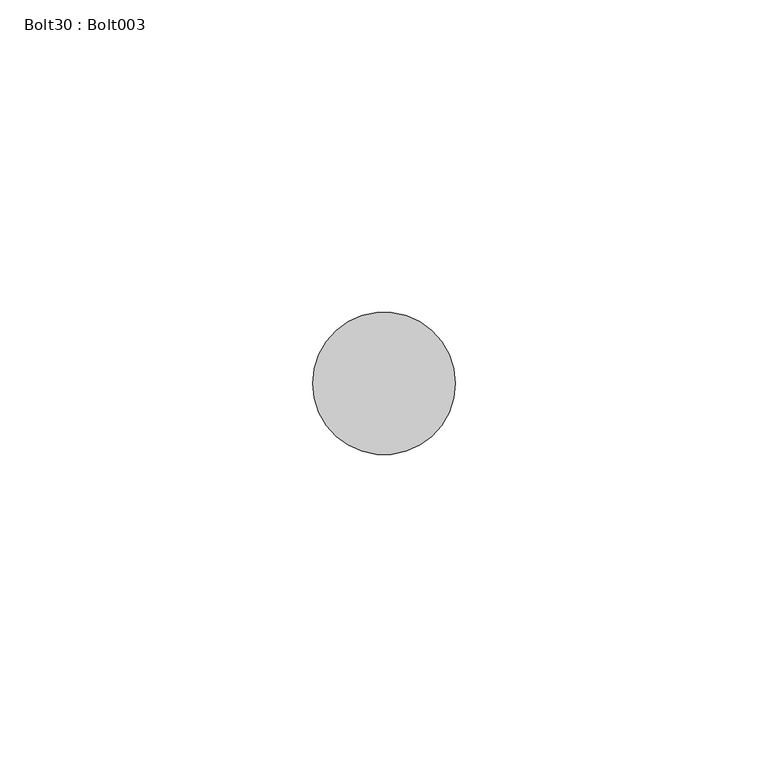
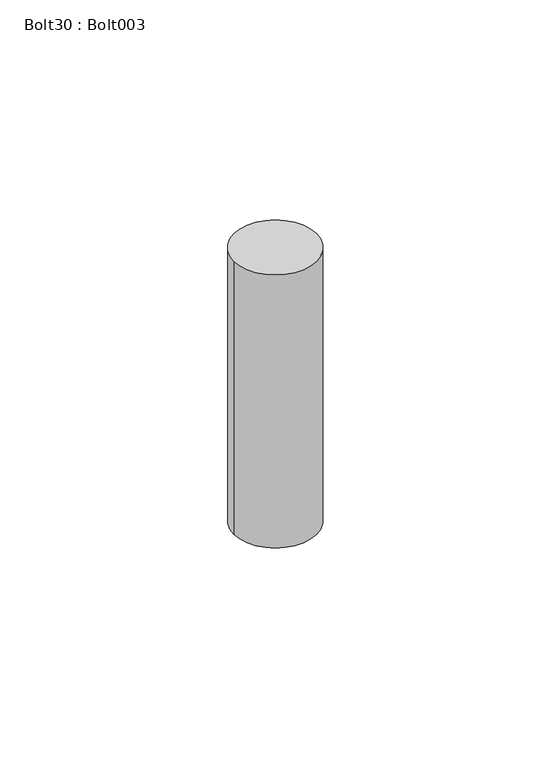
"""IFC4 building model written with IfcOpenShell, lengths in millimetres: proxy geometry, Bolt30 : Bolt003."""

from ifc_helpers import new_model, si_unit, point, frame, frame_2d, origin, place, context, project, spatial, circle_curve, trimmed, segment, composite_curve, outline, extrude, source, transform, mapped, element, save


def bolt30_bolt003_296b5833(model_context):
    return source(origin(), model_context, "Body", "SweptSolid", [
        extrude(outline(composite_curve([segment(trimmed(circle_curve(frame_2d((5172.3828124, 1998.1882072)), 11.4045168), [point((5160.9782956, 1998.1882072))], [point((5183.7873292, 1998.1882072))], False, "CARTESIAN"), True, "CONTINUOUS"), segment(trimmed(circle_curve(frame_2d((5172.3828124, 1998.1882072)), 11.4045168), [point((5183.7873292, 1998.1882072))], [point((5160.9782956, 1998.1882072))], False, "CARTESIAN"), True, "CONTINUOUS")], self_intersect=False)), frame((0.0, 0.0, 36645.5959962), z_axis=(0.0, 0.0, 1.0), x_axis=(1.0, 0.0, 0.0)), (0.0, 0.0, 1.0), 79.375),
    ])


if __name__ == "__main__":
    model = new_model("IFC4")
    model_context = context("Model", 3, world=origin())
    ifc_project = project(units=[si_unit("LENGTHUNIT", "METRE", prefix="MILLI")], contexts=[model_context])
    site = spatial("IfcSite", under=ifc_project)
    building = spatial("IfcBuilding", under=site)
    placement = place(None, origin())
    bolt30_bolt003_shape = bolt30_bolt003_296b5833(model_context)
    element("IfcBuildingElementProxy", 1, Name="Bolt30 : Bolt003", ObjectType="Bolt30 : Bolt003", at=placement, inside=building, context=model_context, shape_type="MappedRepresentation", body=[
        mapped(bolt30_bolt003_shape, transform((0.0, 0.0, 0.0), x_axis=(1.0, 0.0, 0.0), y_axis=(0.0, 1.0, 0.0), z_axis=(0.0, 0.0, 1.0))),
    ])
    save(model, "model.ifc")

# Revit data of these elements
# Type "Bolt30 : Bolt003"
#   NameOverride = "Bolt003"
# Element 1 (IfcBuildingElementProxy, "Bolt30 : Bolt003")
#   Materials on its faces: "STEEL ANGLE AND ANCHOR BOLT (SEE STRUCT. DWGS)"
# Materials
#   "STEEL ANGLE AND ANCHOR BOLT (SEE STRUCT. DWGS)": class "Unassigned", colour RGB 128 128 128, transparency 0, Cost = 0
